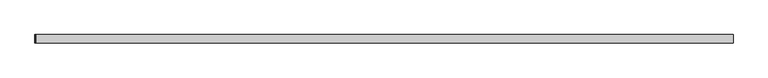
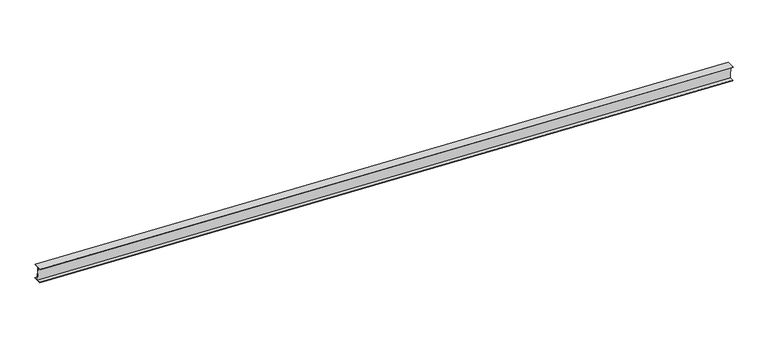
"""IFC4 building model written with IfcOpenShell, lengths in millimetres: proxy geometry, Generic Models 2:Generic Models 2:310765:Generic Models 2:310765 : Generic Models 2:Generic Models 2:310765:198 : Generic Models 2:Generic Models 2:310765:Generic Models 2:310765 : Generic Models 2:Generic Models 2:310765:300385."""

from ifc_helpers import new_model, si_unit, frame, origin, place, context, project, spatial, polyline, outline, extrude, source, transform, mapped, element, save


def generic_models_53026e84(model_context):
    return source(origin(), model_context, "Body", "SweptSolid", [
        extrude(outline(polyline([(6.858, 0.0), (6.858, -73.025), (247.1420001, -73.025), (247.1420001, 0.0), (254.0, 0.0), (254.0, -152.4), (247.1420001, -152.4), (247.1420001, -79.121), (6.858, -79.121), (6.858, -152.4), (0.0, -152.4), (0.0, 0.0), (6.858, 0.0)])), frame((800644.104482, -578474.93331, 3827.1279933), z_axis=(-0.9991330730923567, 0.0, 0.04163054471206784), x_axis=(-0.04163054471206784, 0.0, -0.9991330730923567)), (0.0, 0.0, 1.0), 12411.242059),
    ])


if __name__ == "__main__":
    model = new_model("IFC4")
    model_context = context("Model", 3, world=origin())
    ifc_project = project(units=[si_unit("LENGTHUNIT", "METRE", prefix="MILLI")], contexts=[model_context])
    site = spatial("IfcSite", under=ifc_project)
    building = spatial("IfcBuilding", under=site)
    placement = place(None, origin())
    generic_models_shape = generic_models_53026e84(model_context)
    element("IfcBuildingElementProxy", 1, Name="Generic Models 2:Generic Models 2:310765:Generic Models 2:310765 : Generic Models 2:Generic Models 2:310765:198 : Generic Models 2:Generic Models 2:310765:Generic Models 2:310765 : Generic Models 2:Generic Models 2:310765:300385", ObjectType="Generic Models 2:Generic Models 2:310765:Generic Models 2:310765 : Generic Models 2:Generic Models 2:310765:198 : Generic Models 2:Generic Models 2:310765:Generic Models 2:310765 : Generic Models 2:Generic Models 2:310765:300385", at=placement, inside=building, context=model_context, shape_type="MappedRepresentation", body=[
        mapped(generic_models_shape, transform((0.0, 0.0, 0.0), x_axis=(1.0, 0.0, 0.0), y_axis=(0.0, 1.0, 0.0), z_axis=(0.0, 0.0, 1.0))),
    ])
    save(model, "model.ifc")

# Revit data of these elements
# Type "Generic Models 2:Generic Models 2:310765:Generic Models 2:310765 : Generic Models 2:Generic Models 2:310765:198 : Generic Models 2:Generic Models 2:310765:Generic Models 2:310765 : Generic Models 2:Generic Models 2:310765:300385"
#   NameOverride = "Generic Models 2:Generic Models 2:310765:Generic Models 2:310765 : Generic Models 2:Generic Models 2:310765:300385"
#   ObjectTypeOverride = "Generic Models 2:310765 : Generic Models 2:Generic Models 2:310765"
#   Reference = "Generic Models 2"
#   Tag = "300385"
# Element 1 (IfcBuildingElementProxy, "Generic Models 2:Generic Models 2:310765:Generic Models 2:310765 : Generic Models 2:Generic Models 2:310765:198 : Generic Models 2:Generic Models 2:310765:Generic Models 2:310765 : Generic Models 2:Generic Models 2:310765:300385")
#   Materials on its faces: "THERMAL BROKEN ALUMINUM STOREFRONT FOR POLYCARBONATE"
# Materials
#   "THERMAL BROKEN ALUMINUM STOREFRONT FOR POLYCARBONATE": class "Unassigned", colour RGB 244 244 244, transparency 0, Keynote = "M07611300.01", Cost = 0
